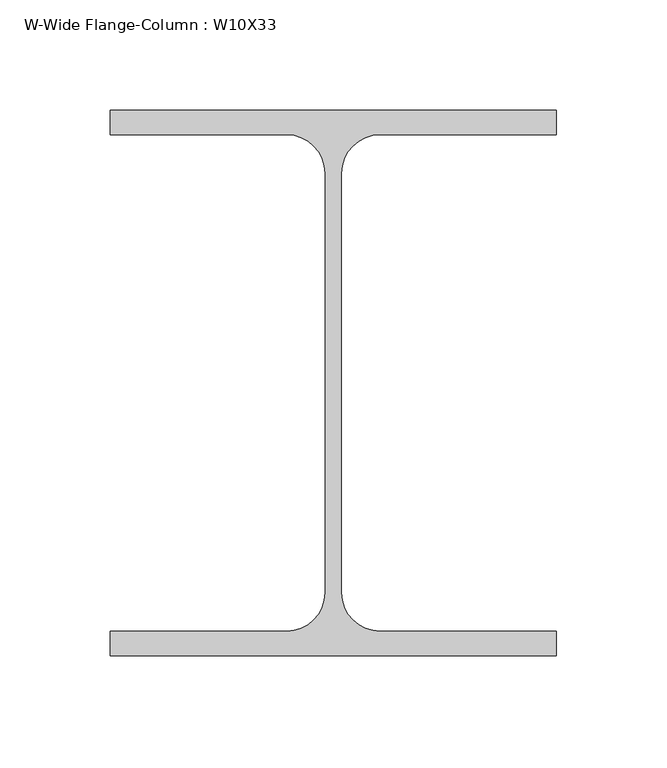
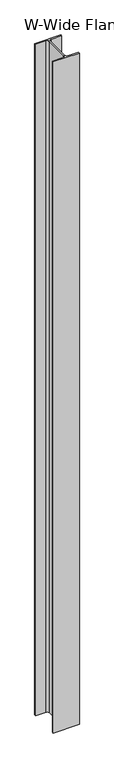
"""IFC4 building model written with IfcOpenShell, lengths in millimetres: column geometry, W-Wide Flange-Column : W10X33."""

from ifc_helpers import new_model, si_unit, point, frame, frame_2d, origin, place, context, project, spatial, polyline, circle_curve, trimmed, segment, composite_curve, outline, extrude, source, transform, mapped, element, save


def w_wide_flange_column_w10x33_d868472c(model_context):
    return source(origin(), model_context, "Body", "SweptSolid", [
        extrude(outline(composite_curve([segment(polyline([(101.092, 123.571), (101.092, 112.522), (21.209, 112.522)]), True, "CONTINUOUS"), segment(trimmed(circle_curve(frame_2d((21.209, 94.996)), 17.526), [point((21.209, 112.522))], [point((3.683, 94.996))], True, "CARTESIAN"), True, "CONTINUOUS"), segment(polyline([(3.683, 94.996), (3.683, -94.996)]), True, "CONTINUOUS"), segment(trimmed(circle_curve(frame_2d((21.209, -94.996)), 17.526), [point((3.683, -94.996))], [point((21.209, -112.522))], True, "CARTESIAN"), True, "CONTINUOUS"), segment(polyline([(21.209, -112.522), (101.092, -112.522), (101.092, -123.571), (-101.092, -123.571), (-101.092, -112.522), (-21.209, -112.522)]), True, "CONTINUOUS"), segment(trimmed(circle_curve(frame_2d((-21.209, -94.996)), 17.526), [point((-21.209, -112.522))], [point((-3.683, -94.996))], True, "CARTESIAN"), True, "CONTINUOUS"), segment(polyline([(-3.683, -94.996), (-3.683, 94.996)]), True, "CONTINUOUS"), segment(trimmed(circle_curve(frame_2d((-21.209, 94.996)), 17.526), [point((-3.683, 94.996))], [point((-21.209, 112.522))], True, "CARTESIAN"), True, "CONTINUOUS"), segment(polyline([(-21.209, 112.522), (-101.092, 112.522), (-101.092, 123.571), (101.092, 123.571)]), True, "CONTINUOUS")], self_intersect=False)), frame((0.0, 0.0, 16408.4), z_axis=(0.0, 0.0, 1.0), x_axis=(1.0, 0.0, 0.0)), (0.0, 0.0, 1.0), 5486.4),
    ])


if __name__ == "__main__":
    model = new_model("IFC4")
    model_context = context("Model", 3, world=origin())
    ifc_project = project(units=[si_unit("LENGTHUNIT", "METRE", prefix="MILLI")], contexts=[model_context])
    site = spatial("IfcSite", under=ifc_project)
    building = spatial("IfcBuilding", under=site)
    placement = place(None, origin())
    w_wide_flange_column_w10x33_shape = w_wide_flange_column_w10x33_d868472c(model_context)
    element("IfcColumn", 1, ObjectType="W-Wide Flange-Column : W10X33", at=placement, inside=building, context=model_context, shape_type="MappedRepresentation", body=[
        mapped(w_wide_flange_column_w10x33_shape, transform((0.0, 0.0, 0.0), x_axis=(1.0, 0.0, 0.0), y_axis=(0.0, 1.0, 0.0), z_axis=(0.0, 0.0, 1.0))),
    ])
    save(model, "model.ifc")

# Revit data of these elements
# Type "W-Wide Flange-Column : W10X33"
#   Assembly Code = "B10"
#   W = 33
#   bf = 0' - 7.96"
#   d = 0' - 9.73"
#   k = 0' - 1 1/8"
#   kr = 0' - 0.69"
#   tf = 0' - 0.435"
#   tw = 0' - 0.29"
#   A = 0.0674306 SF
#   Structural Material [instance default] = Steel ASTM A992
# Element 1 (IfcColumn, "W-Wide Flange-Column : W10X33")
#   Materials on its faces: "Steel ASTM A992"
# Materials
#   "Steel ASTM A992": class "Metal", colour RGB 199 199 199, transparency 0, Description = "Structural steel 50ksi", Cost = 0
